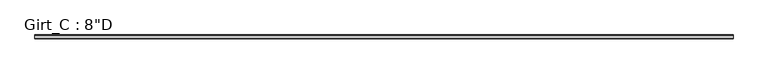
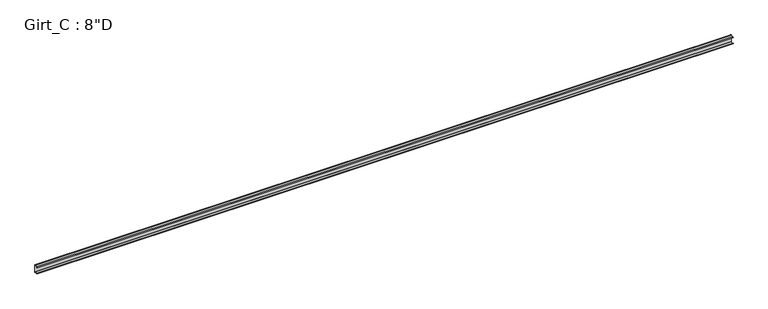
"""IFC4 building model written with IfcOpenShell, lengths in millimetres: beam geometry."""

from ifc_helpers import new_model, si_unit, point, frame, frame_2d, origin, place, context, project, spatial, polyline, circle_curve, trimmed, segment, composite_curve, outline, extrude, source, transform, mapped, element, save


def beam_23314342(model_context):
    return source(origin(), model_context, "Body", "SweptSolid", [
        extrude(outline(composite_curve([segment(polyline([(-87.5109375, 101.6), (-3.3734375, 101.6)]), True, "CONTINUOUS"), segment(trimmed(circle_curve(frame_2d((-3.3734375, 96.8375)), 4.7625), [point((-3.3734375, 101.6))], [point((1.3890625, 96.8375))], False, "CARTESIAN"), True, "CONTINUOUS"), segment(polyline([(1.3890625, 96.8375), (1.3890625, -96.8375)]), True, "CONTINUOUS"), segment(trimmed(circle_curve(frame_2d((-3.3734375, -96.8375)), 4.7625), [point((1.3890625, -96.8375))], [point((-3.3734375, -101.6))], False, "CARTESIAN"), True, "CONTINUOUS"), segment(polyline([(-3.3734375, -101.6), (-87.5109375, -101.6), (-99.7792647, -86.979177), (-97.6510975, -85.1934327), (-86.2154765, -98.821875), (-3.2694106, -98.821875)]), True, "CONTINUOUS"), segment(trimmed(circle_curve(frame_2d((-3.3748024, -96.8389339)), 1.9857399), [point((-3.2694106, -98.821875))], [point((-1.3890625, -96.8389339))], True, "CARTESIAN"), True, "CONTINUOUS"), segment(polyline([(-1.3890625, -96.8389339), (-1.3890625, 96.8381931)]), True, "CONTINUOUS"), segment(trimmed(circle_curve(frame_2d((-3.3741066, 96.8381931)), 1.9850441), [point((-1.3890625, 96.8381931))], [point((-3.3005807, 98.821875))], True, "CARTESIAN"), True, "CONTINUOUS"), segment(polyline([(-3.3005807, 98.821875), (-86.2154765, 98.821875), (-97.6278742, 85.221109), (-99.7560415, 87.0068534), (-87.5109375, 101.6)]), True, "CONTINUOUS")], self_intersect=False)), frame((-9505.9373, 0.0, 0.0), z_axis=(1.0, 0.0, 0.0), x_axis=(0.0, 1.0, 0.0)), (0.0, 0.0, 1.0), 19069.939),
    ])


if __name__ == "__main__":
    model = new_model("IFC4")
    model_context = context("Model", 3, world=origin())
    ifc_project = project(units=[si_unit("LENGTHUNIT", "METRE", prefix="MILLI")], contexts=[model_context])
    site = spatial("IfcSite", under=ifc_project)
    building = spatial("IfcBuilding", under=site)
    placement = place(None, origin())
    beam_shape = beam_23314342(model_context)
    element("IfcBeam", 1, ObjectType="Girt_C : 8\"D", at=placement, inside=building, context=model_context, shape_type="MappedRepresentation", body=[
        mapped(beam_shape, transform((0.0, 0.0, 0.0), x_axis=(1.0, 0.0, 0.0), y_axis=(0.0, 1.0, 0.0), z_axis=(0.0, 0.0, 1.0))),
    ])
    save(model, "model.ifc")

# Revit data of these elements
# Type "Girt_C : 8\"D"
#   half leg = 0' - 1 3/4"
#   Web_Thickness = 0' - 0 7/64"
#   Length [instance default] = 10' - 0"
#   Leg_1 = 0' - 3 1/2"
#   Height = 0' - 8"
#   Structural Material [instance default] = none
# Element 1 (IfcBeam, "Girt_C : 8\"D")
#   Materials on its faces: "CEE' SECTION (8.0x3.5C - SEE STRUCT. DWGS)"
# Materials
#   "CEE' SECTION (8.0x3.5C - SEE STRUCT. DWGS)": class "Metal", colour RGB 137 146 153, transparency 0, Description = "Steel, mill finish", Cost = 0
